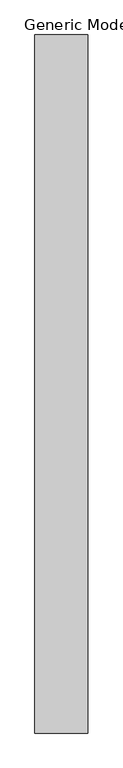
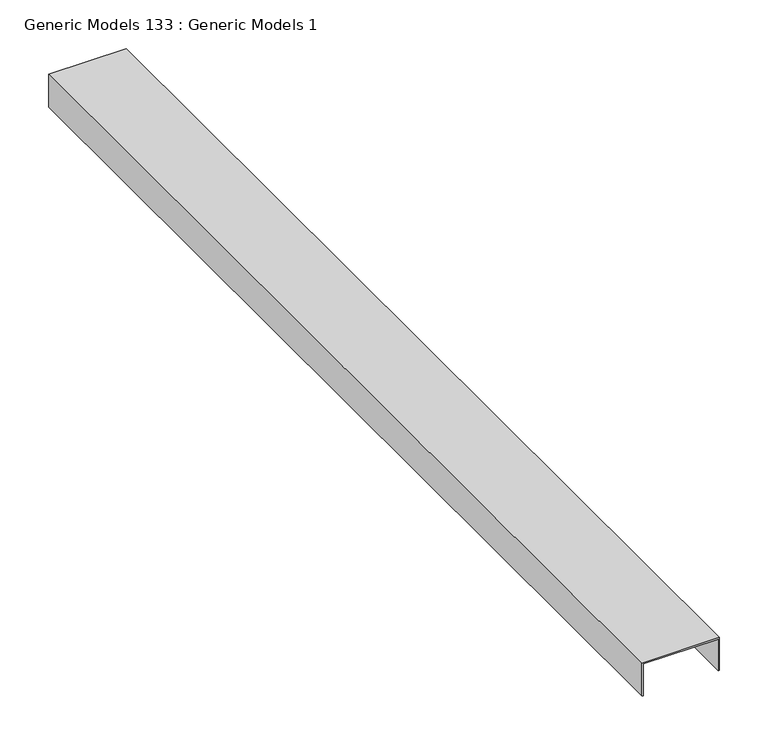
"""IFC4 building model written with IfcOpenShell, lengths in millimetres: proxy geometry, Generic Models 133 : Generic Models 1."""

import ifcopenshell
import ifcopenshell.guid

model = None  # the IFC model being written
_history = None  # IfcOwnerHistory: only IFC2X3 demands one
_inside = {}  # id of a spatial element -> (the spatial element, [elements in it])
_under = {}  # id of a project, library or spatial element -> (it, [spatial elements below it])
_declared = {}  # id of a project -> (the project, [libraries it declares])
_typed = {}  # id of a type object -> (the type object, [elements of that type])
_made_of = {}  # id of a material, layer set ... -> (it, [elements and type objects made of it])


def new_model(schema):
    """Start an empty IFC model of exactly this schema.

    Asked for "IFC4X3", IfcOpenShell would pick the latest addendum, in which some entities
    have other attributes; the version numbers below select the first issue.
    IFC2X3 requires an IfcOwnerHistory on every rooted entity: one is made here for all.
    """
    global model, _history
    if schema == "IFC4X3":
        model = ifcopenshell.file(schema_version=(4, 3, 0, 0))
    else:
        model = ifcopenshell.file(schema=schema)
    _inside.clear()
    _under.clear()
    _declared.clear()
    _typed.clear()
    _made_of.clear()
    _history = None
    if model.schema == "IFC2X3":
        org = make("IfcOrganization", Name="unknown")
        user = make(
            "IfcPersonAndOrganization",
            ThePerson=make("IfcPerson", FamilyName="unknown"),
            TheOrganization=org,
        )
        app = make(
            "IfcApplication",
            ApplicationDeveloper=org,
            Version="unknown",
            ApplicationFullName="unknown",
            ApplicationIdentifier="unknown",
        )
        _history = make(
            "IfcOwnerHistory",
            OwningUser=user,
            OwningApplication=app,
            ChangeAction="ADDED",
            CreationDate=0,
        )
    return model


def make(cls, **values):
    """One entity of the class cls with the attributes given. An attribute that is None is left unset."""
    return model.create_entity(
        cls, **{name: value for name, value in values.items() if value is not None}
    )


def rooted(cls, **values):
    """An entity with a GlobalId (a new one), such as an element, a storey or a relation."""
    return make(cls, GlobalId=ifcopenshell.guid.new(), OwnerHistory=_history, **values)


def si_unit(unit_type, name, prefix=None):
    """IfcSIUnit, for example si_unit("LENGTHUNIT", "METRE", prefix="MILLI")."""
    return make("IfcSIUnit", UnitType=unit_type, Prefix=prefix, Name=name)


def assignment(units):
    """IfcUnitAssignment: the units of a project."""
    return None if units is None else make("IfcUnitAssignment", Units=units)


def point(xyz):
    """IfcCartesianPoint."""
    return None if xyz is None else make("IfcCartesianPoint", Coordinates=xyz)


def direction(xyz):
    """IfcDirection."""
    return None if xyz is None else make("IfcDirection", DirectionRatios=xyz)


def frame(location, z_axis=None, x_axis=None):
    """IfcAxis2Placement3D, a coordinate frame: its origin and axes. An axis left out is left unset."""
    return make(
        "IfcAxis2Placement3D",
        Location=point(location),
        Axis=direction(z_axis),
        RefDirection=direction(x_axis),
    )


def origin():
    """The frame at (0, 0, 0) with its axes left unset."""
    return frame((0.0, 0.0, 0.0))


def place(relative_to, where):
    """IfcLocalPlacement: puts the frame where relative to a parent placement (None: the world)."""
    return make(
        "IfcLocalPlacement", PlacementRelTo=relative_to, RelativePlacement=where
    )


def context(
    kind, dimensions, precision=None, world=None, true_north=None, identifier=None
):
    """IfcGeometricRepresentationContext, for example the 3D "Model" context."""
    return make(
        "IfcGeometricRepresentationContext",
        ContextIdentifier=identifier,
        ContextType=kind,
        CoordinateSpaceDimension=dimensions,
        Precision=precision,
        WorldCoordinateSystem=world,
        TrueNorth=true_north,
    )


def project(units=None, contexts=None):
    """IfcProject with its units and contexts."""
    return rooted(
        "IfcProject",
        Name="project",
        RepresentationContexts=contexts,
        UnitsInContext=assignment(units),
    )


def spatial(cls, under=None, at=None, **own):
    """A site, building, storey or space (cls), placed at a placement, below another one or the project."""
    s = rooted(cls, ObjectPlacement=at, **own)
    if under is not None:
        _under.setdefault(under.id(), (under, []))[1].append(s)
    return s


def polyline(points):
    """IfcPolyline through the points."""
    return make("IfcPolyline", Points=[point(p) for p in points])


def outline(outer, holes=None, kind="AREA"):
    """IfcArbitraryClosedProfileDef: a profile drawn as a closed curve; with holes, ...WithVoids."""
    if holes is None:
        return make("IfcArbitraryClosedProfileDef", ProfileType=kind, OuterCurve=outer)
    return make(
        "IfcArbitraryProfileDefWithVoids",
        ProfileType=kind,
        OuterCurve=outer,
        InnerCurves=holes,
    )


def extrude(swept, where, along, depth):
    """IfcExtrudedAreaSolid: the profile swept, set in the frame where, extruded along a direction by depth."""
    return make(
        "IfcExtrudedAreaSolid",
        SweptArea=swept,
        Position=where,
        ExtrudedDirection=direction(along),
        Depth=depth,
    )


def shape(context_of_items, identifier, shape_type, items):
    """IfcShapeRepresentation: the items that make up one representation, for example the "Body"."""
    return make(
        "IfcShapeRepresentation",
        ContextOfItems=context_of_items,
        RepresentationIdentifier=identifier,
        RepresentationType=shape_type,
        Items=items,
    )


def source(mapping_origin, context_of_items, identifier, shape_type, items):
    """IfcRepresentationMap: a shape defined once, which mapped items show again and again."""
    return make(
        "IfcRepresentationMap",
        MappingOrigin=mapping_origin,
        MappedRepresentation=shape(context_of_items, identifier, shape_type, items),
    )


def transform(
    local_origin,
    x_axis=None,
    y_axis=None,
    z_axis=None,
    scale=None,
    scale2=None,
    scale3=None,
    uniform=True,
):
    """IfcCartesianTransformationOperator3D, or its non-uniform kind. x_axis, y_axis, z_axis: its Axis1, 2, 3."""
    if uniform:
        return make(
            "IfcCartesianTransformationOperator3D",
            Axis1=direction(x_axis),
            Axis2=direction(y_axis),
            LocalOrigin=point(local_origin),
            Scale=scale,
            Axis3=direction(z_axis),
        )
    return make(
        "IfcCartesianTransformationOperator3DnonUniform",
        Axis1=direction(x_axis),
        Axis2=direction(y_axis),
        LocalOrigin=point(local_origin),
        Scale=scale,
        Axis3=direction(z_axis),
        Scale2=scale2,
        Scale3=scale3,
    )


def mapped(mapping_source, mapping_target):
    """IfcMappedItem: shows the shape of a source again, moved by a transform."""
    return make(
        "IfcMappedItem", MappingSource=mapping_source, MappingTarget=mapping_target
    )


def made_of(thing, what):
    """Note that an element or type object is made of a material, layer set ...; save() writes the relation."""
    if what is not None:
        _made_of.setdefault(what.id(), (what, []))[1].append(thing)
    return thing


def element(
    cls,
    number,
    at=None,
    inside=None,
    cuts=None,
    type_object=None,
    material=None,
    context=None,
    identifier="Body",
    shape_type=None,
    held_by="IfcProductDefinitionShape",
    body=None,
    shapes=None,
    **own,
):
    """One element of the class cls, such as IfcWall. Its Tag is "e" and its number.

    at: its placement. inside: the storey or other place that contains it. cuts: it is an
    opening in that element (IfcRelVoidsElement). A single representation is given by context,
    identifier, shape_type and body (its items); several are given by shapes. held_by: the class
    of the entity that holds the representations. save() writes the other relations.
    """
    e = rooted(cls, Tag="e%d" % number, ObjectPlacement=at, **own)
    if body is not None:
        shapes = [shape(context, identifier, shape_type, body)]
    if shapes is not None:
        e.Representation = make(held_by, Representations=shapes)
    if inside is not None:
        _inside.setdefault(inside.id(), (inside, []))[1].append(e)
    if cuts is not None:
        rooted(
            "IfcRelVoidsElement", RelatingBuildingElement=cuts, RelatedOpeningElement=e
        )
    if type_object is not None:
        _typed.setdefault(type_object.id(), (type_object, []))[1].append(e)
    return made_of(e, material)


def aggregate(whole, parts):
    """IfcRelAggregates: a whole, such as a stair, and the parts it consists of."""
    return rooted("IfcRelAggregates", RelatingObject=whole, RelatedObjects=parts)


def save(model, path):
    """Write the relations noted so far, then the file.

    IfcRelAggregates (storeys below a building ...), IfcRelContainedInSpatialStructure (elements
    in a storey), IfcRelDefinesByType, IfcRelAssociatesMaterial and IfcRelDeclares: one each for
    every whole, place, type object, material and project.
    """
    for whole, parts in _under.values():
        aggregate(whole, parts)
    for where, things in _inside.values():
        rooted(
            "IfcRelContainedInSpatialStructure",
            RelatedElements=things,
            RelatingStructure=where,
        )
    for kind, things in _typed.values():
        rooted("IfcRelDefinesByType", RelatedObjects=things, RelatingType=kind)
    for what, things in _made_of.values():
        rooted("IfcRelAssociatesMaterial", RelatedObjects=things, RelatingMaterial=what)
    for by, libraries in _declared.values():
        rooted("IfcRelDeclares", RelatingContext=by, RelatedDefinitions=libraries)
    model.write(path)


def generic_models_133_generic_models_1_467ce512(model_context):
    return source(origin(), model_context, "Body", "SweptSolid", [
        extrude(outline(polyline([(393.2679367, 50793.65), (351.9929367, 50793.65), (351.9929367, 50795.2375), (391.6804367, 50795.2375), (391.6804367, 50884.1375), (351.9929367, 50884.1375), (351.9929367, 50885.725), (393.2679367, 50885.725), (393.2679367, 50793.65)])), frame((0.0, 0.0, 0.0), z_axis=(0.0, 1.0, 0.0), x_axis=(0.0, 0.0, 1.0)), (0.0, 0.0, 1.0), 1219.2),
    ])


if __name__ == "__main__":
    model = new_model("IFC4")
    model_context = context("Model", 3, world=origin())
    ifc_project = project(units=[si_unit("LENGTHUNIT", "METRE", prefix="MILLI")], contexts=[model_context])
    site = spatial("IfcSite", under=ifc_project)
    building = spatial("IfcBuilding", under=site)
    placement = place(None, origin())
    generic_models_133_generic_models_1_shape = generic_models_133_generic_models_1_467ce512(model_context)
    element("IfcBuildingElementProxy", 1, Name="Generic Models 133 : Generic Models 1", ObjectType="Generic Models 133 : Generic Models 1", at=placement, inside=building, context=model_context, shape_type="MappedRepresentation", body=[
        mapped(generic_models_133_generic_models_1_shape, transform((0.0, 0.0, 0.0), x_axis=(1.0, 0.0, 0.0), y_axis=(0.0, 1.0, 0.0), z_axis=(0.0, 0.0, 1.0))),
    ])
    save(model, "model.ifc")

# Revit data of these elements
# Element 1 (IfcBuildingElementProxy, "Generic Models 133 : Generic Models 1")
#   Materials on its faces: "METAL RUNNER ANCHORED TO STRUCTURE"
# Materials
#   "METAL RUNNER ANCHORED TO STRUCTURE": class "Unassigned", colour RGB 210 209 208, transparency 0, Keynote = "M05121300.02", Cost = 0
